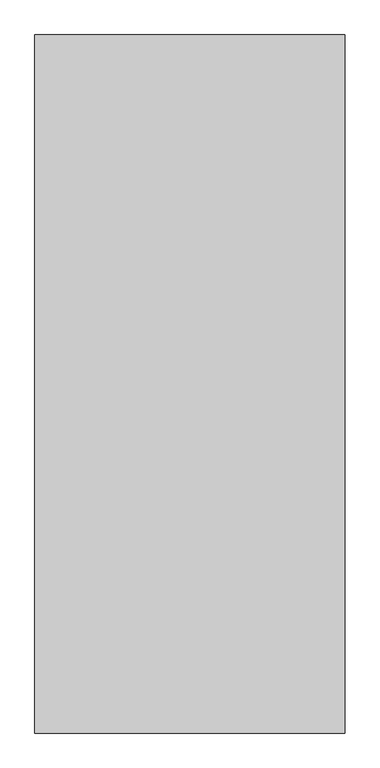
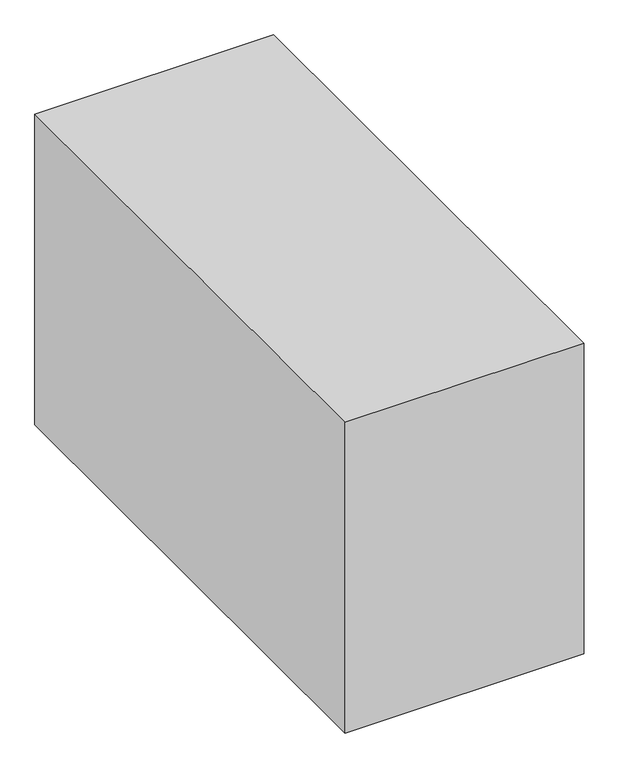
"""IFC4 building model written with IfcOpenShell, lengths in millimetres: proxy geometry, Space Planning Box_hec : Space Planning Box_hec."""

import ifcopenshell
import ifcopenshell.guid

model = None  # the IFC model being written
_history = None  # IfcOwnerHistory: only IFC2X3 demands one
_inside = {}  # id of a spatial element -> (the spatial element, [elements in it])
_under = {}  # id of a project, library or spatial element -> (it, [spatial elements below it])
_declared = {}  # id of a project -> (the project, [libraries it declares])
_typed = {}  # id of a type object -> (the type object, [elements of that type])
_made_of = {}  # id of a material, layer set ... -> (it, [elements and type objects made of it])


def new_model(schema):
    """Start an empty IFC model of exactly this schema.

    Asked for "IFC4X3", IfcOpenShell would pick the latest addendum, in which some entities
    have other attributes; the version numbers below select the first issue.
    IFC2X3 requires an IfcOwnerHistory on every rooted entity: one is made here for all.
    """
    global model, _history
    if schema == "IFC4X3":
        model = ifcopenshell.file(schema_version=(4, 3, 0, 0))
    else:
        model = ifcopenshell.file(schema=schema)
    _inside.clear()
    _under.clear()
    _declared.clear()
    _typed.clear()
    _made_of.clear()
    _history = None
    if model.schema == "IFC2X3":
        org = make("IfcOrganization", Name="unknown")
        user = make(
            "IfcPersonAndOrganization",
            ThePerson=make("IfcPerson", FamilyName="unknown"),
            TheOrganization=org,
        )
        app = make(
            "IfcApplication",
            ApplicationDeveloper=org,
            Version="unknown",
            ApplicationFullName="unknown",
            ApplicationIdentifier="unknown",
        )
        _history = make(
            "IfcOwnerHistory",
            OwningUser=user,
            OwningApplication=app,
            ChangeAction="ADDED",
            CreationDate=0,
        )
    return model


def make(cls, **values):
    """One entity of the class cls with the attributes given. An attribute that is None is left unset."""
    return model.create_entity(
        cls, **{name: value for name, value in values.items() if value is not None}
    )


def rooted(cls, **values):
    """An entity with a GlobalId (a new one), such as an element, a storey or a relation."""
    return make(cls, GlobalId=ifcopenshell.guid.new(), OwnerHistory=_history, **values)


def si_unit(unit_type, name, prefix=None):
    """IfcSIUnit, for example si_unit("LENGTHUNIT", "METRE", prefix="MILLI")."""
    return make("IfcSIUnit", UnitType=unit_type, Prefix=prefix, Name=name)


def assignment(units):
    """IfcUnitAssignment: the units of a project."""
    return None if units is None else make("IfcUnitAssignment", Units=units)


def point(xyz):
    """IfcCartesianPoint."""
    return None if xyz is None else make("IfcCartesianPoint", Coordinates=xyz)


def direction(xyz):
    """IfcDirection."""
    return None if xyz is None else make("IfcDirection", DirectionRatios=xyz)


def frame(location, z_axis=None, x_axis=None):
    """IfcAxis2Placement3D, a coordinate frame: its origin and axes. An axis left out is left unset."""
    return make(
        "IfcAxis2Placement3D",
        Location=point(location),
        Axis=direction(z_axis),
        RefDirection=direction(x_axis),
    )


def origin():
    """The frame at (0, 0, 0) with its axes left unset."""
    return frame((0.0, 0.0, 0.0))


def origin_with_axes():
    """The frame at (0, 0, 0) with the z axis (0, 0, 1) and the x axis (1, 0, 0) written out."""
    return frame((0.0, 0.0, 0.0), z_axis=(0.0, 0.0, 1.0), x_axis=(1.0, 0.0, 0.0))


def place(relative_to, where):
    """IfcLocalPlacement: puts the frame where relative to a parent placement (None: the world)."""
    return make(
        "IfcLocalPlacement", PlacementRelTo=relative_to, RelativePlacement=where
    )


def context(
    kind, dimensions, precision=None, world=None, true_north=None, identifier=None
):
    """IfcGeometricRepresentationContext, for example the 3D "Model" context."""
    return make(
        "IfcGeometricRepresentationContext",
        ContextIdentifier=identifier,
        ContextType=kind,
        CoordinateSpaceDimension=dimensions,
        Precision=precision,
        WorldCoordinateSystem=world,
        TrueNorth=true_north,
    )


def project(units=None, contexts=None):
    """IfcProject with its units and contexts."""
    return rooted(
        "IfcProject",
        Name="project",
        RepresentationContexts=contexts,
        UnitsInContext=assignment(units),
    )


def spatial(cls, under=None, at=None, **own):
    """A site, building, storey or space (cls), placed at a placement, below another one or the project."""
    s = rooted(cls, ObjectPlacement=at, **own)
    if under is not None:
        _under.setdefault(under.id(), (under, []))[1].append(s)
    return s


def polyline(points):
    """IfcPolyline through the points."""
    return make("IfcPolyline", Points=[point(p) for p in points])


def outline(outer, holes=None, kind="AREA"):
    """IfcArbitraryClosedProfileDef: a profile drawn as a closed curve; with holes, ...WithVoids."""
    if holes is None:
        return make("IfcArbitraryClosedProfileDef", ProfileType=kind, OuterCurve=outer)
    return make(
        "IfcArbitraryProfileDefWithVoids",
        ProfileType=kind,
        OuterCurve=outer,
        InnerCurves=holes,
    )


def extrude(swept, where, along, depth):
    """IfcExtrudedAreaSolid: the profile swept, set in the frame where, extruded along a direction by depth."""
    return make(
        "IfcExtrudedAreaSolid",
        SweptArea=swept,
        Position=where,
        ExtrudedDirection=direction(along),
        Depth=depth,
    )


def shape(context_of_items, identifier, shape_type, items):
    """IfcShapeRepresentation: the items that make up one representation, for example the "Body"."""
    return make(
        "IfcShapeRepresentation",
        ContextOfItems=context_of_items,
        RepresentationIdentifier=identifier,
        RepresentationType=shape_type,
        Items=items,
    )


def source(mapping_origin, context_of_items, identifier, shape_type, items):
    """IfcRepresentationMap: a shape defined once, which mapped items show again and again."""
    return make(
        "IfcRepresentationMap",
        MappingOrigin=mapping_origin,
        MappedRepresentation=shape(context_of_items, identifier, shape_type, items),
    )


def transform(
    local_origin,
    x_axis=None,
    y_axis=None,
    z_axis=None,
    scale=None,
    scale2=None,
    scale3=None,
    uniform=True,
):
    """IfcCartesianTransformationOperator3D, or its non-uniform kind. x_axis, y_axis, z_axis: its Axis1, 2, 3."""
    if uniform:
        return make(
            "IfcCartesianTransformationOperator3D",
            Axis1=direction(x_axis),
            Axis2=direction(y_axis),
            LocalOrigin=point(local_origin),
            Scale=scale,
            Axis3=direction(z_axis),
        )
    return make(
        "IfcCartesianTransformationOperator3DnonUniform",
        Axis1=direction(x_axis),
        Axis2=direction(y_axis),
        LocalOrigin=point(local_origin),
        Scale=scale,
        Axis3=direction(z_axis),
        Scale2=scale2,
        Scale3=scale3,
    )


def mapped(mapping_source, mapping_target):
    """IfcMappedItem: shows the shape of a source again, moved by a transform."""
    return make(
        "IfcMappedItem", MappingSource=mapping_source, MappingTarget=mapping_target
    )


def made_of(thing, what):
    """Note that an element or type object is made of a material, layer set ...; save() writes the relation."""
    if what is not None:
        _made_of.setdefault(what.id(), (what, []))[1].append(thing)
    return thing


def element(
    cls,
    number,
    at=None,
    inside=None,
    cuts=None,
    type_object=None,
    material=None,
    context=None,
    identifier="Body",
    shape_type=None,
    held_by="IfcProductDefinitionShape",
    body=None,
    shapes=None,
    **own,
):
    """One element of the class cls, such as IfcWall. Its Tag is "e" and its number.

    at: its placement. inside: the storey or other place that contains it. cuts: it is an
    opening in that element (IfcRelVoidsElement). A single representation is given by context,
    identifier, shape_type and body (its items); several are given by shapes. held_by: the class
    of the entity that holds the representations. save() writes the other relations.
    """
    e = rooted(cls, Tag="e%d" % number, ObjectPlacement=at, **own)
    if body is not None:
        shapes = [shape(context, identifier, shape_type, body)]
    if shapes is not None:
        e.Representation = make(held_by, Representations=shapes)
    if inside is not None:
        _inside.setdefault(inside.id(), (inside, []))[1].append(e)
    if cuts is not None:
        rooted(
            "IfcRelVoidsElement", RelatingBuildingElement=cuts, RelatedOpeningElement=e
        )
    if type_object is not None:
        _typed.setdefault(type_object.id(), (type_object, []))[1].append(e)
    return made_of(e, material)


def aggregate(whole, parts):
    """IfcRelAggregates: a whole, such as a stair, and the parts it consists of."""
    return rooted("IfcRelAggregates", RelatingObject=whole, RelatedObjects=parts)


def save(model, path):
    """Write the relations noted so far, then the file.

    IfcRelAggregates (storeys below a building ...), IfcRelContainedInSpatialStructure (elements
    in a storey), IfcRelDefinesByType, IfcRelAssociatesMaterial and IfcRelDeclares: one each for
    every whole, place, type object, material and project.
    """
    for whole, parts in _under.values():
        aggregate(whole, parts)
    for where, things in _inside.values():
        rooted(
            "IfcRelContainedInSpatialStructure",
            RelatedElements=things,
            RelatingStructure=where,
        )
    for kind, things in _typed.values():
        rooted("IfcRelDefinesByType", RelatedObjects=things, RelatingType=kind)
    for what, things in _made_of.values():
        rooted("IfcRelAssociatesMaterial", RelatedObjects=things, RelatingMaterial=what)
    for by, libraries in _declared.values():
        rooted("IfcRelDeclares", RelatingContext=by, RelatedDefinitions=libraries)
    model.write(path)


def generic_models_8934d72c(model_context):
    return source(origin(), model_context, "Body", "SweptSolid", [
        extrude(outline(polyline([(2000.0, 4500.0), (2000.0, -4500.0), (-2000.0, -4500.0), (-2000.0, 4500.0), (2000.0, 4500.0)])), origin_with_axes(), (0.0, 0.0, 1.0), 5500.0),
    ])


if __name__ == "__main__":
    model = new_model("IFC4")
    model_context = context("Model", 3, world=origin())
    ifc_project = project(units=[si_unit("LENGTHUNIT", "METRE", prefix="MILLI")], contexts=[model_context])
    site = spatial("IfcSite", under=ifc_project)
    building = spatial("IfcBuilding", under=site)
    placement = place(None, origin())
    generic_models_shape = generic_models_8934d72c(model_context)
    element("IfcBuildingElementProxy", 1, Name="Space Planning Box_hec : Space Planning Box_hec", ObjectType="Space Planning Box_hec : Space Planning Box_hec", at=placement, inside=building, context=model_context, shape_type="MappedRepresentation", body=[
        mapped(generic_models_shape, transform((0.0, 0.0, 0.0), x_axis=(1.0, 0.0, 0.0), y_axis=(0.0, 1.0, 0.0), z_axis=(0.0, 0.0, 1.0))),
    ])
    save(model, "model.ifc")

# Revit data of these elements
# Type "Space Planning Box_hec : Space Planning Box_hec"
#   Type Comments = "..."
#   Room Name [instance default] = "?"
#   Interior Finish [instance default] = ""
#   Exterior Finish [instance default] = ""
#   Department [instance default] = ""
#   Assembly Code = "..."
#   ceiling height [instance default] = 0
#   Width [instance default] = 1524 mm
#   Program Area [instance default] = 0.00 m²
#   Length [instance default] = 1524 mm
#   Height [instance default] = 1524 mm
#   Area [instance default] = 2.32258 m²
#   Fill Color [instance default] = Cyan
#   Default Elevation = 0
# Element 1 (IfcBuildingElementProxy, "Space Planning Box_hec : Space Planning Box_hec")
#   Room Name = "Lobby"
#   Exterior Finish = "N/A..N/A,,EW2..N/A..N/A"
#   Department = "AR"
#   Width = 4000 mm
#   Program Area = 36.00 m²
#   Length = 9000 mm
#   Height = 5500 mm
#   Area = 36.00 m²
#   Materials on its faces: "Cyan"
# Materials
#   "Cyan": class "Generic", colour RGB 0 255 255, transparency 0.2, Cost = 0
